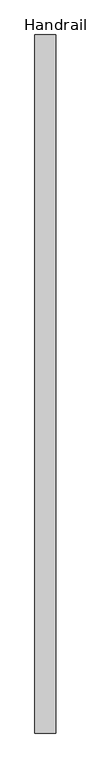
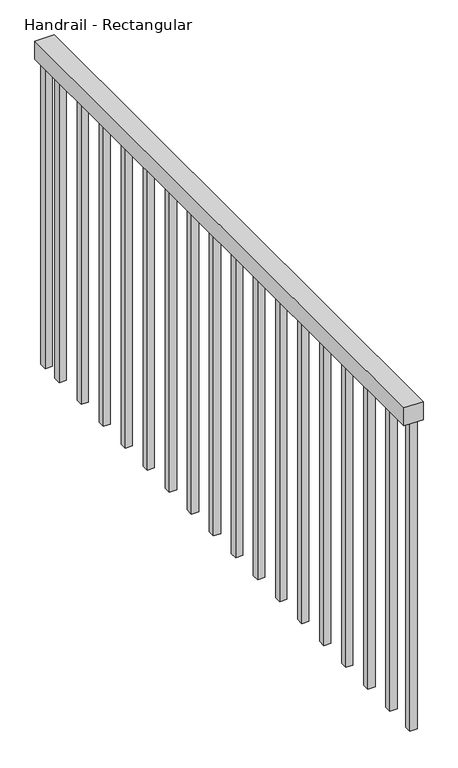
"""IFC4 building model written with IfcOpenShell, lengths in millimetres: railing geometry, Handrail - Rectangular."""

from ifc_helpers import new_model, si_unit, frame, origin, place, context, project, spatial, polyline, outline, extrude, source, transform, mapped, element, save


def handrail_rectangular_1c66f9c2(model_context):
    return source(origin(), model_context, "Body", "SweptSolid", [
        extrude(outline(polyline([(-12364.4211091, 745.8507146), (-12415.2211091, 745.8507146), (-12415.2211091, 2445.8507146), (-12364.4211091, 2445.8507146), (-12364.4211091, 745.8507146)])), frame((0.0, 0.0, 6654.4), z_axis=(0.0, 0.0, 1.0), x_axis=(1.0, 0.0, 0.0)), (0.0, 0.0, 1.0), 50.8),
        extrude(outline(polyline([(-12380.2961091, 2361.9257146), (-12399.3461091, 2361.9257146), (-12399.3461091, 2380.9757146), (-12380.2961091, 2380.9757146), (-12380.2961091, 2361.9257146)])), frame((0.0, 0.0, 5790.8), z_axis=(0.0, 0.0, 1.0), x_axis=(1.0, 0.0, 0.0)), (0.0, 0.0, 1.0), 863.6),
        extrude(outline(polyline([(-12380.2961091, 2260.3257146), (-12399.3461091, 2260.3257146), (-12399.3461091, 2279.3757146), (-12380.2961091, 2279.3757146), (-12380.2961091, 2260.3257146)])), frame((0.0, 0.0, 5790.8), z_axis=(0.0, 0.0, 1.0), x_axis=(1.0, 0.0, 0.0)), (0.0, 0.0, 1.0), 863.6),
        extrude(outline(polyline([(-12380.2961091, 2158.7257146), (-12399.3461091, 2158.7257146), (-12399.3461091, 2177.7757146), (-12380.2961091, 2177.7757146), (-12380.2961091, 2158.7257146)])), frame((0.0, 0.0, 5790.8), z_axis=(0.0, 0.0, 1.0), x_axis=(1.0, 0.0, 0.0)), (0.0, 0.0, 1.0), 863.6),
        extrude(outline(polyline([(-12380.2961091, 2057.1257146), (-12399.3461091, 2057.1257146), (-12399.3461091, 2076.1757146), (-12380.2961091, 2076.1757146), (-12380.2961091, 2057.1257146)])), frame((0.0, 0.0, 5790.8), z_axis=(0.0, 0.0, 1.0), x_axis=(1.0, 0.0, 0.0)), (0.0, 0.0, 1.0), 863.6),
        extrude(outline(polyline([(-12380.2961091, 1955.5257146), (-12399.3461091, 1955.5257146), (-12399.3461091, 1974.5757146), (-12380.2961091, 1974.5757146), (-12380.2961091, 1955.5257146)])), frame((0.0, 0.0, 5790.8), z_axis=(0.0, 0.0, 1.0), x_axis=(1.0, 0.0, 0.0)), (0.0, 0.0, 1.0), 863.6),
        extrude(outline(polyline([(-12380.2961091, 1853.9257146), (-12399.3461091, 1853.9257146), (-12399.3461091, 1872.9757146), (-12380.2961091, 1872.9757146), (-12380.2961091, 1853.9257146)])), frame((0.0, 0.0, 5790.8), z_axis=(0.0, 0.0, 1.0), x_axis=(1.0, 0.0, 0.0)), (0.0, 0.0, 1.0), 863.6),
        extrude(outline(polyline([(-12380.2961091, 1752.3257146), (-12399.3461091, 1752.3257146), (-12399.3461091, 1771.3757146), (-12380.2961091, 1771.3757146), (-12380.2961091, 1752.3257146)])), frame((0.0, 0.0, 5790.8), z_axis=(0.0, 0.0, 1.0), x_axis=(1.0, 0.0, 0.0)), (0.0, 0.0, 1.0), 863.6),
        extrude(outline(polyline([(-12380.2961091, 1650.7257146), (-12399.3461091, 1650.7257146), (-12399.3461091, 1669.7757146), (-12380.2961091, 1669.7757146), (-12380.2961091, 1650.7257146)])), frame((0.0, 0.0, 5790.8), z_axis=(0.0, 0.0, 1.0), x_axis=(1.0, 0.0, 0.0)), (0.0, 0.0, 1.0), 863.6),
        extrude(outline(polyline([(-12380.2961091, 1549.1257146), (-12399.3461091, 1549.1257146), (-12399.3461091, 1568.1757146), (-12380.2961091, 1568.1757146), (-12380.2961091, 1549.1257146)])), frame((0.0, 0.0, 5790.8), z_axis=(0.0, 0.0, 1.0), x_axis=(1.0, 0.0, 0.0)), (0.0, 0.0, 1.0), 863.6),
        extrude(outline(polyline([(-12380.2961091, 1447.5257146), (-12399.3461091, 1447.5257146), (-12399.3461091, 1466.5757146), (-12380.2961091, 1466.5757146), (-12380.2961091, 1447.5257146)])), frame((0.0, 0.0, 5790.8), z_axis=(0.0, 0.0, 1.0), x_axis=(1.0, 0.0, 0.0)), (0.0, 0.0, 1.0), 863.6),
        extrude(outline(polyline([(-12380.2961091, 1345.9257146), (-12399.3461091, 1345.9257146), (-12399.3461091, 1364.9757146), (-12380.2961091, 1364.9757146), (-12380.2961091, 1345.9257146)])), frame((0.0, 0.0, 5790.8), z_axis=(0.0, 0.0, 1.0), x_axis=(1.0, 0.0, 0.0)), (0.0, 0.0, 1.0), 863.6),
        extrude(outline(polyline([(-12380.2961091, 1244.3257146), (-12399.3461091, 1244.3257146), (-12399.3461091, 1263.3757146), (-12380.2961091, 1263.3757146), (-12380.2961091, 1244.3257146)])), frame((0.0, 0.0, 5790.8), z_axis=(0.0, 0.0, 1.0), x_axis=(1.0, 0.0, 0.0)), (0.0, 0.0, 1.0), 863.6),
        extrude(outline(polyline([(-12380.2961091, 1142.7257146), (-12399.3461091, 1142.7257146), (-12399.3461091, 1161.7757146), (-12380.2961091, 1161.7757146), (-12380.2961091, 1142.7257146)])), frame((0.0, 0.0, 5790.8), z_axis=(0.0, 0.0, 1.0), x_axis=(1.0, 0.0, 0.0)), (0.0, 0.0, 1.0), 863.6),
        extrude(outline(polyline([(-12380.2961091, 1041.1257146), (-12399.3461091, 1041.1257146), (-12399.3461091, 1060.1757146), (-12380.2961091, 1060.1757146), (-12380.2961091, 1041.1257146)])), frame((0.0, 0.0, 5790.8), z_axis=(0.0, 0.0, 1.0), x_axis=(1.0, 0.0, 0.0)), (0.0, 0.0, 1.0), 863.6),
        extrude(outline(polyline([(-12380.2961091, 939.5257146), (-12399.3461091, 939.5257146), (-12399.3461091, 958.5757146), (-12380.2961091, 958.5757146), (-12380.2961091, 939.5257146)])), frame((0.0, 0.0, 5790.8), z_axis=(0.0, 0.0, 1.0), x_axis=(1.0, 0.0, 0.0)), (0.0, 0.0, 1.0), 863.6),
        extrude(outline(polyline([(-12380.2961091, 837.9257146), (-12399.3461091, 837.9257146), (-12399.3461091, 856.9757146), (-12380.2961091, 856.9757146), (-12380.2961091, 837.9257146)])), frame((0.0, 0.0, 5790.8), z_axis=(0.0, 0.0, 1.0), x_axis=(1.0, 0.0, 0.0)), (0.0, 0.0, 1.0), 863.6),
        extrude(outline(polyline([(-12380.2961091, 2426.8007146), (-12399.3461091, 2426.8007146), (-12399.3461091, 2445.8507146), (-12380.2961091, 2445.8507146), (-12380.2961091, 2426.8007146)])), frame((0.0, 0.0, 5790.8), z_axis=(0.0, 0.0, 1.0), x_axis=(1.0, 0.0, 0.0)), (0.0, 0.0, 1.0), 863.6),
        extrude(outline(polyline([(-12380.2961091, 745.8507146), (-12399.3461091, 745.8507146), (-12399.3461091, 764.9007146), (-12380.2961091, 764.9007146), (-12380.2961091, 745.8507146)])), frame((0.0, 0.0, 5790.8), z_axis=(0.0, 0.0, 1.0), x_axis=(1.0, 0.0, 0.0)), (0.0, 0.0, 1.0), 863.6),
    ])


if __name__ == "__main__":
    model = new_model("IFC4")
    model_context = context("Model", 3, world=origin())
    ifc_project = project(units=[si_unit("LENGTHUNIT", "METRE", prefix="MILLI")], contexts=[model_context])
    site = spatial("IfcSite", under=ifc_project)
    building = spatial("IfcBuilding", under=site)
    placement = place(None, origin())
    handrail_rectangular_shape = handrail_rectangular_1c66f9c2(model_context)
    element("IfcRailing", 1, ObjectType="Handrail - Rectangular", at=placement, inside=building, context=model_context, shape_type="MappedRepresentation", body=[
        mapped(handrail_rectangular_shape, transform((0.0, 0.0, 0.0), x_axis=(1.0, 0.0, 0.0), y_axis=(0.0, 1.0, 0.0), z_axis=(0.0, 0.0, 1.0))),
    ])
    save(model, "model.ifc")
